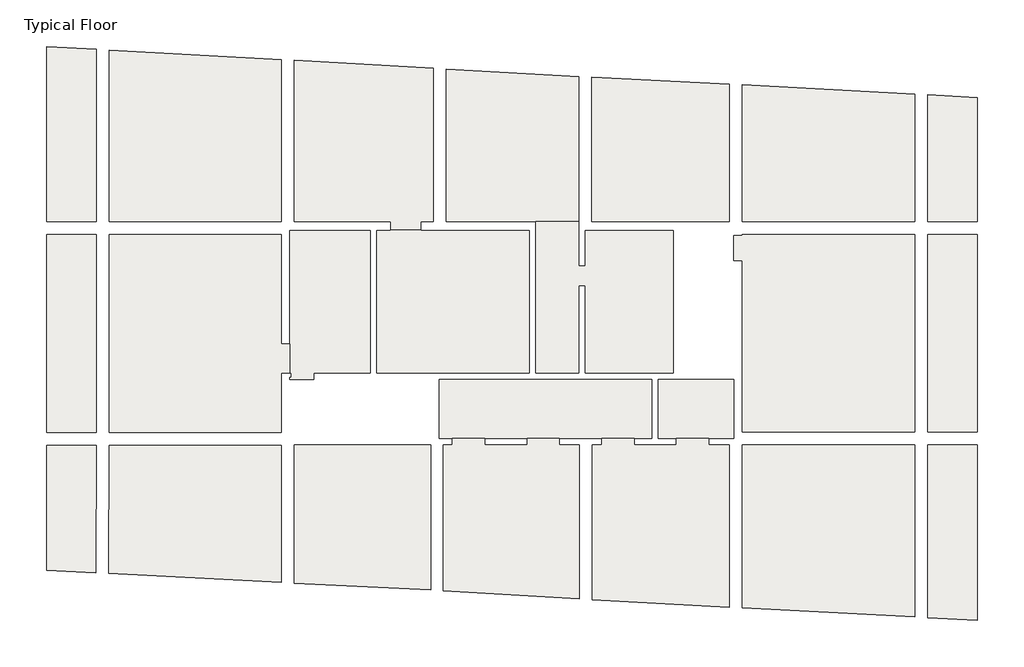
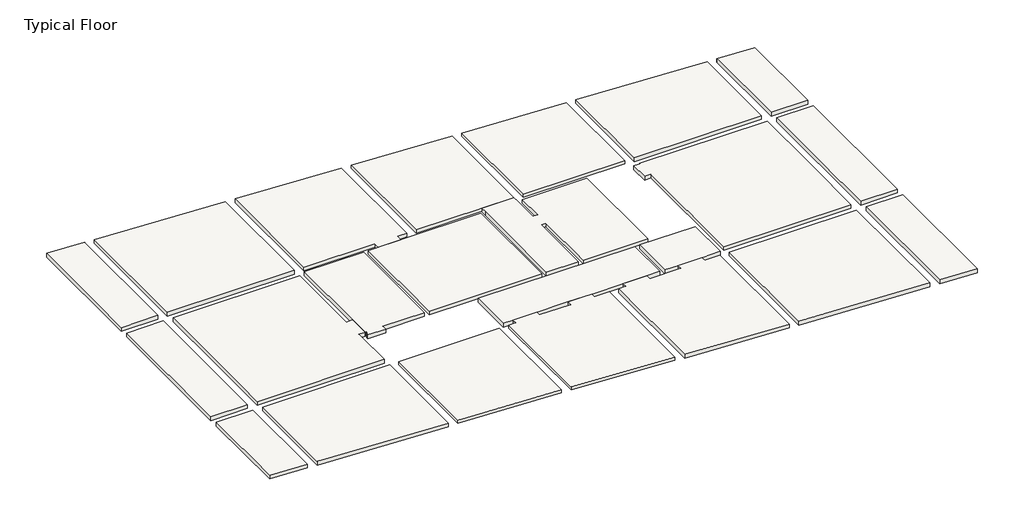
# One storey: 23 slabs.
"""IFC4 building model written with IfcOpenShell, lengths in millimetres."""

from ifc_helpers import new_model, si_unit, frame, origin, place, context, project, spatial, polyline, outline, extrude, faceted_brep, element, save

model = new_model("IFC4")

# Units and contexts
model_context = context("Model", 3, world=origin())
ifc_project = project(units=[si_unit("LENGTHUNIT", "METRE", prefix="MILLI")], contexts=[model_context])

# Site, building, storey
site = spatial("IfcSite", under=ifc_project)
building = spatial("IfcBuilding", under=site)
storey = spatial("IfcBuildingStorey", under=building, Name="Typical Floor", Elevation=3500.0)

# Slabs
placement = place(None, origin())
element("IfcSlab", 1, ObjectType="20", at=placement, inside=storey, context=model_context, shape_type="Brep", body=[
    faceted_brep([(-702.7226745, -8172.2965545, 3300.0), (-702.7226745, -14884.028101, 3300.0), (-6997.0277588, -14575.1203917, 3300.0), (-6997.0277588, -8172.2965545, 3300.0), (-702.7226745, -8172.2965545, 3500.0), (-6997.0277588, -8172.2965545, 3500.0), (-6997.0277588, -14560.7582621, 3500.0), (-6997.0277588, -14575.1203917, 3500.0), (-702.7226745, -14884.028101, 3500.0)], [[[0, 1, 2, 3]], [[4, 5, 6, 7, 8]], [[1, 0, 4, 8]], [[2, 1, 8, 7]], [[3, 2, 7, 6, 5]], [[0, 3, 5, 4]]]),
])
element("IfcSlab", 2, ObjectType="20", at=placement, inside=storey, context=model_context, shape_type="Brep", body=[
    faceted_brep([(-102.7226745, -8172.2965545, 3300.0), (309.3899821, -8172.2965545, 3300.0), (309.3899821, -7872.2965545, 3300.0), (1808.0058991, -7872.2965545, 3300.0), (1808.0058991, -8172.2965545, 3300.0), (3757.0255069, -8172.2965545, 3300.0), (3757.0255069, -7872.2965545, 3300.0), (5255.6414239, -7872.2965545, 3300.0), (5255.6414239, -8172.2965545, 3300.0), (6172.0250706, -8172.2965545, 3300.0), (6172.0250706, -15300.3845543, 3300.0), (-102.7226745, -14916.8878336, 3300.0), (309.3899821, -8172.2965545, 3500.0), (-102.7226745, -8172.2965545, 3500.0), (-102.7226745, -14899.1123715, 3500.0), (-102.7226745, -14916.8878336, 3500.0), (6172.0250706, -15300.3845543, 3500.0), (6172.0250706, -8172.2965545, 3500.0), (5255.6414239, -8172.2965545, 3500.0), (5255.6414239, -7872.2965545, 3500.0), (3757.0255069, -7872.2965545, 3500.0), (3757.0255069, -8172.2965545, 3500.0), (1808.0058991, -8172.2965545, 3500.0), (1808.0058991, -7872.2965545, 3500.0), (309.3899821, -7872.2965545, 3500.0)], [[[0, 1, 2, 3, 4, 5, 6, 7, 8, 9, 10, 11]], [[12, 13, 14, 15, 16, 17, 18, 19, 20, 21, 22, 23, 24]], [[1, 0, 13, 12]], [[2, 1, 12, 24]], [[3, 2, 24, 23]], [[4, 3, 23, 22]], [[5, 4, 22, 21]], [[6, 5, 21, 20]], [[7, 6, 20, 19]], [[8, 7, 19, 18]], [[9, 8, 18, 17]], [[10, 9, 17, 16]], [[11, 10, 16, 15]], [[0, 11, 15, 14, 13]]]),
])
element("IfcSlab", 3, ObjectType="20", at=placement, inside=storey, context=model_context, shape_type="Brep", body=[
    faceted_brep([(6756.4488056, 8818.2924867, 3300.0), (13105.5837537, 8500.9277886, 3300.0), (13105.5837537, 2137.8533878, 3300.0), (6756.4488056, 2137.8533878, 3300.0), (6756.4488056, 8818.2924867, 3500.0), (6756.4488056, 2137.8533878, 3500.0), (13105.5837537, 2137.8533878, 3500.0), (13105.5837537, 8486.6836559, 3500.0), (13105.5837537, 8500.9277886, 3500.0)], [[[0, 1, 2, 3]], [[4, 5, 6, 7, 8]], [[1, 0, 4, 8]], [[2, 1, 8, 7, 6]], [[3, 2, 6, 5]], [[0, 3, 5, 4]]]),
])
element("IfcSlab", 4, ObjectType="20", at=placement, inside=storey, context=model_context, shape_type="Brep", body=[
    faceted_brep([(33.1500744, 9202.9682104, 3300.0), (6156.4488056, 8850.5502029, 3300.0), (6156.4488056, 2137.8533878, 3300.0), (4155.2954031, 2137.8533878, 3300.0), (33.1500744, 2137.8533878, 3300.0), (33.1500744, 9202.9682104, 3500.0), (33.1500744, 2137.8533878, 3500.0), (4155.2954031, 2137.8533878, 3500.0), (4158.2942497, 2137.8533878, 3500.0), (6156.4488056, 2137.8533878, 3500.0), (6156.4488056, 8832.8840986, 3500.0), (6156.4488056, 8850.5502029, 3500.0)], [[[0, 1, 2, 3, 4]], [[5, 6, 7, 8, 9, 10, 11]], [[1, 0, 5, 11]], [[2, 1, 11, 10, 9]], [[4, 3, 7, 6]], [[0, 4, 6, 5]], [[3, 2, 9, 8, 7]]]),
])
element("IfcSlab", 5, ObjectType="25", at=placement, inside=storey, context=model_context, shape_type="Brep", body=[
    faceted_brep([(-7599.5626242, 9632.0768029, 3250.0), (-7599.5626242, 2137.8533878, 3250.0), (-15545.0048536, 2137.8533878, 3250.0), (-15536.4663265, 10078.6836364, 3250.0), (-7599.5626242, 9632.0768029, 3500.0), (-15536.4663265, 10078.6836364, 3500.0), (-15545.0048536, 2137.8533878, 3500.0), (-7599.5626242, 2137.8533878, 3500.0), (-7599.5626242, 9596.3425232, 3500.0)], [[[0, 1, 2, 3]], [[4, 5, 6, 7, 8]], [[1, 0, 4, 8, 7]], [[2, 1, 7, 6]], [[3, 2, 6, 5]], [[0, 3, 5, 4]]]),
])
element("IfcSlab", 6, ObjectType="25", at=placement, inside=storey, context=model_context, shape_type="Brep", body=[
    faceted_brep([(-16136.4303725, 10112.4434063, 3250.0), (-16145.0052005, 2137.8533878, 3250.0), (-18443.7818749, 2137.8533878, 3250.0), (-18443.7818749, 10242.2772794, 3250.0), (-16136.4303725, 10112.4434063, 3500.0), (-18443.7818749, 10242.2772794, 3500.0), (-18443.7818749, 2137.8533878, 3500.0), (-16145.0052005, 2137.8533878, 3500.0), (-16136.4525662, 10091.8032303, 3500.0)], [[[0, 1, 2, 3]], [[4, 5, 6, 7, 8]], [[1, 0, 4, 8, 7]], [[2, 1, 7, 6]], [[3, 2, 6, 5]], [[0, 3, 5, 4]]]),
])
element("IfcSlab", 7, ObjectType="25", at=placement, inside=storey, context=model_context, shape_type="Brep", body=[
    faceted_brep([(-16155.474628, -7598.714204, 3250.0), (-18443.7818749, -7598.714204, 3250.0), (-18443.7818749, 1537.8533878, 3250.0), (-16145.6503618, 1537.8533878, 3250.0), (-16150.3278096, -2812.1730545, 3250.0), (-16150.9729705, -3412.1727076, 3250.0), (-16155.4742813, -7598.391797, 3250.0), (-18443.7818749, -7598.714204, 3500.0), (-16155.474628, -7598.714204, 3500.0), (-16155.4742813, -7598.391797, 3500.0), (-16150.9729705, -3412.1727076, 3500.0), (-16150.3278096, -2812.1730545, 3500.0), (-16145.6503618, 1537.8533878, 3500.0), (-18443.7818749, 1537.8533878, 3500.0)], [[[0, 1, 2, 3, 4, 5, 6]], [[7, 8, 9, 10, 11, 12, 13]], [[8, 0, 6, 5, 4, 3, 12, 11, 10, 9]], [[1, 0, 8, 7]], [[2, 1, 7, 13]], [[3, 2, 13, 12]]]),
])
element("IfcSlab", 8, ObjectType="25", at=placement, inside=storey, context=model_context, shape_type="SweptSolid", body=[
    extrude(outline(polyline([(-18443.7818749, -8198.714204), (-16156.1197893, -8198.714204), (-16162.4537125, -14089.2628163), (-18443.7818749, -13968.0424313), (-18443.7818749, -8198.714204)])), frame((0.0, 0.0, 3250.0), z_axis=(0.0, 0.0, 1.0), x_axis=(1.0, 0.0, 0.0)), (0.0, 0.0, 1.0), 250.0),
])
element("IfcSlab", 9, ObjectType="25", at=placement, inside=storey, context=model_context, shape_type="Brep", body=[
    faceted_brep([(-7597.0277588, -14544.3942826, 3250.0), (-15562.4876449, -14121.1425427, 3250.0), (-15556.1197891, -8199.036611, 3250.0), (-15556.1194424, -8198.714204, 3250.0), (-7597.0277588, -8198.714204, 3250.0), (-15562.4876449, -14121.1425427, 3500.0), (-7597.0277588, -14544.3942826, 3500.0), (-7597.0277588, -8198.714204, 3500.0), (-15556.1194424, -8198.714204, 3500.0), (-15556.1197891, -8199.036611, 3500.0), (-15562.471289, -14105.9314844, 3500.0)], [[[0, 1, 2, 3, 4]], [[5, 6, 7, 8, 9, 10]], [[1, 0, 6, 5]], [[1, 5, 10, 9, 8, 3, 2]], [[4, 3, 8, 7]], [[0, 4, 7, 6]]]),
])
element("IfcSlab", 10, ObjectType="25", at=placement, inside=storey, context=model_context, shape_type="Brep", body=[
    faceted_brep([(-7599.5626242, 1537.8533878, 3250.0), (-7599.5626242, -3512.6656433, 3250.0), (-7199.5626242, -3512.6656433, 3250.0), (-7199.5626242, -4855.687558, 3250.0), (-7599.5626242, -4855.687558, 3250.0), (-7599.5626242, -5055.687558, 3250.0), (-7599.5626242, -7598.714204, 3250.0), (-15555.4742811, -7598.714204, 3250.0), (-15550.9733173, -3412.8178686, 3250.0), (-15550.3281564, -2812.8182154, 3250.0), (-15545.6500149, 1537.8533878, 3250.0), (-7599.5626242, -3512.6656433, 3500.0), (-7599.5626242, 1537.8533878, 3500.0), (-15545.0119134, 1537.8533878, 3500.0), (-15545.6500149, 1537.8533878, 3500.0), (-15550.3281564, -2812.8182154, 3500.0), (-15550.9733173, -3412.8178686, 3500.0), (-15555.4742811, -7598.714204, 3500.0), (-7599.5626242, -7598.714204, 3500.0), (-7599.5626242, -5055.687558, 3500.0), (-7599.5626242, -4855.687558, 3500.0), (-7199.5626242, -4855.687558, 3500.0), (-7199.5626242, -3512.6656433, 3500.0)], [[[0, 1, 2, 3, 4, 5, 6, 7, 8, 9, 10]], [[11, 12, 13, 14, 15, 16, 17, 18, 19, 20, 21, 22]], [[1, 0, 12, 11]], [[2, 1, 11, 22]], [[3, 2, 22, 21]], [[4, 3, 21, 20]], [[4, 20, 19, 18, 6, 5]], [[7, 6, 18, 17]], [[7, 17, 16, 15, 14, 10, 9, 8]], [[0, 10, 14, 13, 12]]]),
])
element("IfcSlab", 11, ObjectType="25", at=placement, inside=storey, context=model_context, shape_type="Brep", body=[
    faceted_brep([(-3490.3793374, 1737.8533878, 3250.0), (-3490.3793374, -4855.687558, 3250.0), (-6094.5315865, -4855.687558, 3250.0), (-6094.5315865, -5155.687558, 3250.0), (-7199.5626242, -5155.687558, 3250.0), (-7199.5626242, -5055.687558, 3250.0), (-7139.5626242, -5055.687558, 3250.0), (-7139.5626242, -4855.687558, 3250.0), (-7199.5626242, -4855.687558, 3250.0), (-7199.5626242, -3512.6656433, 3250.0), (-7199.5626242, 1737.8533878, 3250.0), (-3490.3793374, -4855.687558, 3500.0), (-3490.3793374, 1737.8533878, 3500.0), (-7199.5626242, 1737.8533878, 3500.0), (-7199.5626242, -3512.6656433, 3500.0), (-7199.5626242, -4855.687558, 3500.0), (-7139.5626242, -4855.687558, 3500.0), (-7139.5626242, -5055.687558, 3500.0), (-7199.5626242, -5055.687558, 3500.0), (-7199.5626242, -5155.687558, 3500.0), (-6094.5315865, -5155.687558, 3500.0), (-6094.5315865, -4855.687558, 3500.0)], [[[0, 1, 2, 3, 4, 5, 6, 7, 8, 9, 10]], [[11, 12, 13, 14, 15, 16, 17, 18, 19, 20, 21]], [[1, 0, 12, 11]], [[2, 1, 11, 21]], [[3, 2, 21, 20]], [[4, 3, 20, 19]], [[5, 4, 19, 18]], [[6, 5, 18, 17]], [[7, 6, 17, 16]], [[8, 7, 16, 15]], [[10, 9, 8, 15, 14, 13]], [[0, 10, 13, 12]]]),
])
element("IfcSlab", 12, ObjectType="25", at=placement, inside=storey, context=model_context, shape_type="Brep", body=[
    faceted_brep([(6772.0250706, -8172.2965545, 3250.0), (7204.6610317, -8172.2965545, 3250.0), (7204.6610317, -7872.2965545, 3250.0), (8703.2769487, -7872.2965545, 3250.0), (8703.2769487, -8172.2965545, 3250.0), (10652.2965565, -8172.2965545, 3250.0), (10652.2965565, -7872.2965545, 3250.0), (12150.9124735, -7872.2965545, 3250.0), (12150.9124735, -8172.2965545, 3250.0), (13105.5837537, -8172.2965545, 3250.0), (13105.5837537, -15690.2789818, 3250.0), (6772.0250706, -15335.6091222, 3250.0), (7204.6610317, -8172.2965545, 3500.0), (6772.0250706, -8172.2965545, 3500.0), (6772.0250706, -15319.2795755, 3500.0), (6772.0250706, -15335.6091222, 3500.0), (13105.5837537, -15690.2789818, 3500.0), (13105.5837537, -8172.2965545, 3500.0), (12150.9124735, -8172.2965545, 3500.0), (12150.9124735, -7872.2965545, 3500.0), (10652.2965565, -7872.2965545, 3500.0), (10652.2965565, -8172.2965545, 3500.0), (8703.2769487, -8172.2965545, 3500.0), (8703.2769487, -7872.2965545, 3500.0), (7204.6610317, -7872.2965545, 3500.0)], [[[0, 1, 2, 3, 4, 5, 6, 7, 8, 9, 10, 11]], [[12, 13, 14, 15, 16, 17, 18, 19, 20, 21, 22, 23, 24]], [[1, 0, 13, 12]], [[2, 1, 12, 24]], [[3, 2, 24, 23]], [[4, 3, 23, 22]], [[5, 4, 22, 21]], [[6, 5, 21, 20]], [[7, 6, 20, 19]], [[8, 7, 19, 18]], [[9, 8, 18, 17]], [[10, 9, 17, 16]], [[11, 10, 16, 15]], [[0, 11, 15, 14, 13]]]),
])
element("IfcSlab", 13, ObjectType="25", at=placement, inside=storey, context=model_context, shape_type="Brep", body=[
    faceted_brep([(9530.3819083, -5155.687558, 3250.0), (9530.3819083, -7872.2965545, 3250.0), (8703.2769487, -7872.2965545, 3250.0), (7204.6610317, -7872.2965545, 3250.0), (-291.6077111, -7872.2965545, 3250.0), (-291.6077111, -5155.687558, 3250.0), (9530.3819083, -5155.687558, 3500.0), (-291.6077111, -5155.687558, 3500.0), (-291.6077111, -7872.2965545, 3500.0), (309.3899821, -7872.2965545, 3500.0), (1808.0058991, -7872.2965545, 3500.0), (3757.0255069, -7872.2965545, 3500.0), (5255.6414239, -7872.2965545, 3500.0), (7204.6610317, -7872.2965545, 3500.0), (8703.2769487, -7872.2965545, 3500.0), (9530.3819083, -7872.2965545, 3500.0)], [[[0, 1, 2, 3, 4, 5]], [[6, 7, 8, 9, 10, 11, 12, 13, 14, 15]], [[1, 0, 6, 15]], [[4, 3, 2, 1, 15, 14, 13, 12, 11, 10, 9, 8]], [[5, 4, 8, 7]], [[0, 5, 7, 6]]]),
])
element("IfcSlab", 14, ObjectType="25", at=placement, inside=storey, context=model_context, shape_type="Brep", body=[
    faceted_brep([(13305.5837537, -5155.687558, 3250.0), (13305.5837537, -7872.2965545, 3250.0), (12150.9124735, -7872.2965545, 3250.0), (10652.2965565, -7872.2965545, 3250.0), (9830.3819083, -7872.2965545, 3250.0), (9830.3819083, -5155.687558, 3250.0), (13305.5837537, -5155.687558, 3500.0), (9830.3819083, -5155.687558, 3500.0), (9830.3819083, -7872.2965545, 3500.0), (10652.2965565, -7872.2965545, 3500.0), (12150.9124735, -7872.2965545, 3500.0), (13305.5837537, -7872.2965545, 3500.0)], [[[0, 1, 2, 3, 4, 5]], [[6, 7, 8, 9, 10, 11]], [[1, 0, 6, 11]], [[4, 3, 2, 1, 11, 10, 9, 8]], [[5, 4, 8, 7]], [[0, 5, 7, 6]]]),
])
element("IfcSlab", 15, ObjectType="25", at=placement, inside=storey, context=model_context, shape_type="Brep", body=[
    faceted_brep([(13305.5837537, 1490.9099045, 3250.0), (13705.5837537, 1490.9099045, 3250.0), (13705.5837537, 1537.8533878, 3250.0), (21672.320563, 1537.8533878, 3250.0), (21672.320563, -7572.2965545, 3250.0), (13705.5837537, -7572.2965545, 3250.0), (13705.5837537, 336.2386242, 3250.0), (13305.5837537, 336.2386242, 3250.0), (13705.5837537, 1490.9099045, 3500.0), (13305.5837537, 1490.9099045, 3500.0), (13305.5837537, 336.2386242, 3500.0), (13705.5837537, 336.2386242, 3500.0), (13705.5837537, -7572.2965545, 3500.0), (21672.320563, -7572.2965545, 3500.0), (21672.320563, -3412.4954615, 3500.0), (21672.320563, -2812.4954615, 3500.0), (21672.320563, 1537.8533878, 3500.0), (13705.5837537, 1537.8533878, 3500.0)], [[[0, 1, 2, 3, 4, 5, 6, 7]], [[8, 9, 10, 11, 12, 13, 14, 15, 16, 17]], [[1, 0, 9, 8]], [[2, 1, 8, 17]], [[3, 2, 17, 16]], [[4, 3, 16, 15, 14, 13]], [[5, 4, 13, 12]], [[6, 5, 12, 11]], [[7, 6, 11, 10]], [[0, 7, 10, 9]]]),
])
element("IfcSlab", 16, ObjectType="25", at=placement, inside=storey, context=model_context, shape_type="SweptSolid", body=[
    extrude(outline(polyline([(13705.5837537, -8172.2965545), (21672.320563, -8172.2965545), (21672.320563, -16132.9877815), (13705.5837537, -15722.5717744), (13705.5837537, -8172.2965545)])), frame((0.0, 0.0, 3250.0), z_axis=(0.0, 0.0, 1.0), x_axis=(1.0, 0.0, 0.0)), (0.0, 0.0, 1.0), 250.0),
])
element("IfcSlab", 17, ObjectType="25", at=placement, inside=storey, context=model_context, shape_type="Brep", body=[
    faceted_brep([(24568.7448881, -16282.2005564, 3250.0), (22272.320563, -16163.8975015, 3250.0), (22272.320563, -8172.2965545, 3250.0), (24568.7448881, -8172.2965545, 3250.0), (24568.7448881, -16282.2005564, 3500.0), (24568.7448881, -8172.2965545, 3500.0), (22272.320563, -8172.2965545, 3500.0), (22272.320563, -16148.8404655, 3500.0), (22272.320563, -16163.8975015, 3500.0)], [[[0, 1, 2, 3]], [[4, 5, 6, 7, 8]], [[1, 0, 4, 8]], [[2, 1, 8, 7, 6]], [[3, 2, 6, 5]], [[0, 3, 5, 4]]]),
])
element("IfcSlab", 18, ObjectType="25", at=placement, inside=storey, context=model_context, shape_type="Brep", body=[
    faceted_brep([(24568.7448881, 1537.8533878, 3250.0), (24568.7448881, -7572.2965545, 3250.0), (22272.320563, -7572.2965545, 3250.0), (22272.320563, 1537.8533878, 3250.0), (24568.7448881, 1537.8533878, 3500.0), (22272.320563, 1537.8533878, 3500.0), (22272.320563, -2812.4954615, 3500.0), (22272.320563, -3412.4954615, 3500.0), (22272.320563, -7572.2965545, 3500.0), (24568.7448881, -7572.2965545, 3500.0)], [[[0, 1, 2, 3]], [[4, 5, 6, 7, 8, 9]], [[1, 0, 4, 9]], [[2, 1, 9, 8]], [[3, 2, 8, 7, 6, 5]], [[0, 3, 5, 4]]]),
])
element("IfcSlab", 19, ObjectType="25", at=placement, inside=storey, context=model_context, shape_type="SweptSolid", body=[
    extrude(outline(polyline([(24568.7448881, 2137.8533878), (22272.320563, 2137.8533878), (22272.320563, 7998.3813629), (22272.7386809, 7998.381946), (22272.7208607, 8011.159025), (24568.7448881, 7885.5038131), (24568.7448881, 2137.8533878)])), frame((0.0, 0.0, 3250.0), z_axis=(0.0, 0.0, 1.0), x_axis=(1.0, 0.0, 0.0)), (0.0, 0.0, 1.0), 250.0),
])
element("IfcSlab", 20, ObjectType="25", at=placement, inside=storey, context=model_context, shape_type="Brep", body=[
    faceted_brep([(10507.8905588, 1737.8533878, 3250.0), (10507.8905588, -4855.687558, 3250.0), (6456.4488056, -4855.687558, 3250.0), (6456.4488056, -810.243498, 3250.0), (6156.4488056, -810.243498, 3250.0), (6156.4488056, -4855.687558, 3250.0), (4155.2954031, -4855.687558, 3250.0), (4155.2954031, 1737.8533878, 3250.0), (4158.2942497, 1737.8533878, 3250.0), (4158.2942497, 2137.8533878, 3250.0), (6156.4488056, 2137.8533878, 3250.0), (6156.4488056, 1737.8533878, 3250.0), (6156.4488056, 90.5638838, 3250.0), (6456.4488056, 90.5638838, 3250.0), (6456.4488056, 1737.8533878, 3250.0), (10507.8905588, -4855.687558, 3500.0), (10507.8905588, 1737.8533878, 3500.0), (6456.4488056, 1737.8533878, 3500.0), (6456.4488056, 90.5638838, 3500.0), (6156.4488056, 90.5638838, 3500.0), (6156.4488056, 1737.8533878, 3500.0), (6156.4488056, 2137.8533878, 3500.0), (4158.2942497, 2137.8533878, 3500.0), (4158.2942497, 1737.8533878, 3500.0), (4155.2954031, 1737.8533878, 3500.0), (4155.2954031, -4855.687558, 3500.0), (6156.4488056, -4855.687558, 3500.0), (6156.4488056, -810.243498, 3500.0), (6456.4488056, -810.243498, 3500.0), (6456.4488056, -4855.687558, 3500.0), (6156.4488056, 2137.8533878, 3300.0)], [[[0, 1, 2, 3, 4, 5, 6, 7, 8, 9, 10, 11, 12, 13, 14]], [[15, 16, 17, 18, 19, 20, 21, 22, 23, 24, 25, 26, 27, 28, 29]], [[1, 0, 16, 15]], [[2, 1, 15, 29]], [[3, 2, 29, 28]], [[0, 14, 17, 16]], [[4, 3, 28, 27]], [[5, 4, 27, 26]], [[6, 5, 26, 25]], [[6, 25, 24, 7]], [[21, 30, 10, 9, 22]], [[10, 30, 21, 20, 19, 12, 11]], [[13, 12, 19, 18]], [[14, 13, 18, 17]], [[23, 8, 7, 24]], [[8, 23, 22, 9]]]),
])
element("IfcSlab", 21, ObjectType="25", at=placement, inside=storey, context=model_context, shape_type="SweptSolid", body=[
    extrude(outline(polyline([(3855.2954031, -4855.687558), (-3190.3793374, -4855.687558), (-3190.3793374, 1737.8533878), (-2548.6261655, 1737.8533878), (-2548.6261655, 1752.8533878), (-1148.2801448, 1752.8533878), (-1148.2801448, 1737.8533878), (3855.2954031, 1737.8533878), (3855.2954031, -4855.687558)])), frame((0.0, 0.0, 3250.0), z_axis=(0.0, 0.0, 1.0), x_axis=(1.0, 0.0, 0.0)), (0.0, 0.0, 1.0), 250.0),
])
element("IfcSlab", 22, ObjectType="25", at=placement, inside=storey, context=model_context, shape_type="SweptSolid", body=[
    extrude(outline(polyline([(13705.5837537, 8480.0153679), (21672.320563, 8044.0173164), (21672.320563, 2137.8533878), (13705.5837537, 2137.8533878), (13705.5837537, 8480.0153679)])), frame((0.0, 0.0, 3250.0), z_axis=(0.0, 0.0, 1.0), x_axis=(1.0, 0.0, 0.0)), (0.0, 0.0, 1.0), 250.0),
])
element("IfcSlab", 23, ObjectType="25", at=placement, inside=storey, context=model_context, shape_type="Brep", body=[
    faceted_brep([(-566.8499256, 9237.1370793, 3250.0), (-566.8499256, 2137.8533878, 3250.0), (-1148.2801448, 2137.8533878, 3250.0), (-1148.2801448, 1752.8533878, 3250.0), (-2548.6261655, 1752.8533878, 3250.0), (-2548.6261655, 2137.8533878, 3250.0), (-6999.5626242, 2137.8533878, 3250.0), (-6999.5626242, 9599.1036038, 3250.0), (-566.8499256, 2137.8533878, 3500.0), (-566.8499256, 9220.7307485, 3500.0), (-566.8499256, 9237.1370793, 3500.0), (-6999.5626242, 9599.1036038, 3500.0), (-6999.5626242, 9596.3425232, 3500.0), (-6999.5626242, 2137.8533878, 3500.0), (-2548.6261655, 2137.8533878, 3500.0), (-2548.6261655, 1752.8533878, 3500.0), (-1148.2801448, 1752.8533878, 3500.0), (-1148.2801448, 2137.8533878, 3500.0)], [[[0, 1, 2, 3, 4, 5, 6, 7]], [[8, 9, 10, 11, 12, 13, 14, 15, 16, 17]], [[1, 0, 10, 9, 8]], [[2, 1, 8, 17]], [[2, 17, 16, 3]], [[14, 5, 4, 15]], [[6, 5, 14, 13]], [[7, 6, 13, 12, 11]], [[0, 7, 11, 10]], [[4, 3, 16, 15]]]),
])

save(model, "model.ifc")

# Revit data of these elements
# Type "20"
#   Function = 0
#   Layers, outside or top first: 20 cm "Concrete" (function 1)
# Type "25"
#   Function = 0
#   Layers, outside or top first: 25 cm "Concrete" (function 1)
# Element 1 (IfcSlab, "20")
#   Mark = "S20"
#   SOFiSTiK_AMG_Comments = ""
#   Height Offset From Level = 0 cm
#   built-in parameter 1001954 = 1
#   SOFiSTiK_AMG_Scheduled = yes
#   SOFiSTiK_AMG_Adjusted = yes
#   Phase Created = New Construction
#   Materials on its faces: "Concrete"
# Element 2 (IfcSlab, "20")
#   Mark = "S21"
#   SOFiSTiK_AMG_Comments = ""
#   built-in parameter 1001955 = 1.5708 (stored number, unit not read)
#   Height Offset From Level = 0 cm
#   built-in parameter 1001954 = 1
#   SOFiSTiK_AMG_Scheduled = yes
#   SOFiSTiK_AMG_Adjusted = yes
#   Phase Created = New Construction
#   Materials on its faces: "Concrete"
# Element 3 (IfcSlab, "20")
#   Mark = "S22"
#   SOFiSTiK_AMG_Comments = ""
#   built-in parameter 1001955 = 1.5708 (stored number, unit not read)
#   Height Offset From Level = 0 cm
#   built-in parameter 1001954 = 1
#   SOFiSTiK_AMG_Scheduled = yes
#   SOFiSTiK_AMG_Adjusted = yes
#   Phase Created = New Construction
#   Materials on its faces: "Concrete"
# Element 4 (IfcSlab, "20")
#   Mark = "S23"
#   SOFiSTiK_AMG_Comments = ""
#   built-in parameter 1001955 = 1.5708 (stored number, unit not read)
#   Height Offset From Level = 0 cm
#   built-in parameter 1001954 = 1
#   SOFiSTiK_AMG_Scheduled = yes
#   SOFiSTiK_AMG_Adjusted = yes
#   Phase Created = New Construction
#   Materials on its faces: "Concrete"
# Element 5 (IfcSlab, "25")
#   Mark = "S1"
#   SOFiSTiK_AMG_Comments = ""
#   built-in parameter 1001955 = -0.0562104 (stored number, unit not read)
#   Height Offset From Level = 0 cm
#   built-in parameter 1001954 = 1
#   SOFiSTiK_AMG_Scheduled = yes
#   SOFiSTiK_AMG_Adjusted = yes
#   Phase Created = New Construction
#   Materials on its faces: "Concrete"
# Element 6 (IfcSlab, "25")
#   Mark = "S2"
#   SOFiSTiK_AMG_Comments = ""
#   built-in parameter 1001955 = -0.0562104 (stored number, unit not read)
#   Height Offset From Level = 0 cm
#   built-in parameter 1001954 = 1
#   SOFiSTiK_AMG_Scheduled = yes
#   SOFiSTiK_AMG_Adjusted = yes
#   Phase Created = New Construction
#   Materials on its faces: "Concrete"
# Element 7 (IfcSlab, "25")
#   Mark = "S3"
#   SOFiSTiK_AMG_Comments = ""
#   Height Offset From Level = 0 cm
#   built-in parameter 1001954 = 1
#   SOFiSTiK_AMG_Scheduled = yes
#   SOFiSTiK_AMG_Adjusted = yes
#   Phase Created = New Construction
#   Materials on its faces: "Concrete"
# Element 8 (IfcSlab, "25")
#   Mark = "S4"
#   SOFiSTiK_AMG_Comments = ""
#   built-in parameter 1001955 = 1.5708 (stored number, unit not read)
#   Height Offset From Level = 0 cm
#   built-in parameter 1001954 = 1
#   SOFiSTiK_AMG_Scheduled = yes
#   SOFiSTiK_AMG_Adjusted = yes
#   Phase Created = New Construction
#   Materials on its faces: "Concrete"
# Element 9 (IfcSlab, "25")
#   Mark = "S5"
#   SOFiSTiK_AMG_Comments = ""
#   built-in parameter 1001955 = -0.053086 (stored number, unit not read)
#   Height Offset From Level = 0 cm
#   built-in parameter 1001954 = 1
#   SOFiSTiK_AMG_Scheduled = yes
#   SOFiSTiK_AMG_Adjusted = yes
#   Phase Created = New Construction
#   Materials on its faces: "Concrete"
# Element 10 (IfcSlab, "25")
#   Mark = "S6"
#   SOFiSTiK_AMG_Comments = ""
#   Height Offset From Level = 0 cm
#   built-in parameter 1001954 = 1
#   SOFiSTiK_AMG_Scheduled = yes
#   SOFiSTiK_AMG_Adjusted = yes
#   Phase Created = New Construction
#   Materials on its faces: "Concrete"
# Element 11 (IfcSlab, "25")
#   Mark = "S7"
#   SOFiSTiK_AMG_Comments = ""
#   Height Offset From Level = 0 cm
#   built-in parameter 1001954 = 1
#   SOFiSTiK_AMG_Scheduled = yes
#   SOFiSTiK_AMG_Adjusted = yes
#   Phase Created = New Construction
#   Materials on its faces: "Concrete"
# Element 12 (IfcSlab, "25")
#   Mark = "S8"
#   SOFiSTiK_AMG_Comments = ""
#   built-in parameter 1001955 = 1.5708 (stored number, unit not read)
#   Height Offset From Level = 0 cm
#   built-in parameter 1001954 = 1
#   SOFiSTiK_AMG_Scheduled = yes
#   SOFiSTiK_AMG_Adjusted = yes
#   Phase Created = New Construction
#   Materials on its faces: "Concrete"
# Element 13 (IfcSlab, "25")
#   Mark = "S9"
#   SOFiSTiK_AMG_Comments = ""
#   Height Offset From Level = 0 cm
#   built-in parameter 1001954 = 1
#   SOFiSTiK_AMG_Scheduled = yes
#   SOFiSTiK_AMG_Adjusted = yes
#   Phase Created = New Construction
#   Materials on its faces: "Concrete"
# Element 14 (IfcSlab, "25")
#   Mark = "S10"
#   SOFiSTiK_AMG_Comments = ""
#   Height Offset From Level = 0 cm
#   built-in parameter 1001954 = 1
#   SOFiSTiK_AMG_Scheduled = yes
#   SOFiSTiK_AMG_Adjusted = yes
#   Phase Created = New Construction
#   Materials on its faces: "Concrete"
# Element 15 (IfcSlab, "25")
#   Mark = "S11"
#   SOFiSTiK_AMG_Comments = ""
#   built-in parameter 1001955 = 1.5708 (stored number, unit not read)
#   Height Offset From Level = 0 cm
#   built-in parameter 1001954 = 1
#   SOFiSTiK_AMG_Scheduled = yes
#   SOFiSTiK_AMG_Adjusted = yes
#   Phase Created = New Construction
#   Materials on its faces: "Concrete"
# Element 16 (IfcSlab, "25")
#   Mark = "S12"
#   SOFiSTiK_AMG_Comments = ""
#   built-in parameter 1001955 = 1.5708 (stored number, unit not read)
#   Height Offset From Level = 0 cm
#   built-in parameter 1001954 = 1
#   SOFiSTiK_AMG_Scheduled = yes
#   SOFiSTiK_AMG_Adjusted = yes
#   Phase Created = New Construction
#   Materials on its faces: "Concrete"
# Element 17 (IfcSlab, "25")
#   Mark = "S13"
#   SOFiSTiK_AMG_Comments = ""
#   built-in parameter 1001955 = -0.0514707 (stored number, unit not read)
#   Height Offset From Level = 0 cm
#   built-in parameter 1001954 = 1
#   SOFiSTiK_AMG_Scheduled = yes
#   SOFiSTiK_AMG_Adjusted = yes
#   Phase Created = New Construction
#   Materials on its faces: "Concrete"
# Element 18 (IfcSlab, "25")
#   Mark = "S14"
#   SOFiSTiK_AMG_Comments = ""
#   Height Offset From Level = 0 cm
#   built-in parameter 1001954 = 1
#   SOFiSTiK_AMG_Scheduled = yes
#   SOFiSTiK_AMG_Adjusted = yes
#   Phase Created = New Construction
#   Materials on its faces: "Concrete"
# Element 19 (IfcSlab, "25")
#   Mark = "S15"
#   SOFiSTiK_AMG_Comments = ""
#   built-in parameter 1001955 = -1.5708 (stored number, unit not read)
#   Height Offset From Level = 0 cm
#   built-in parameter 1001954 = 1
#   SOFiSTiK_AMG_Scheduled = yes
#   SOFiSTiK_AMG_Adjusted = yes
#   Phase Created = New Construction
#   Materials on its faces: "Concrete"
# Element 20 (IfcSlab, "25")
#   Mark = "S16"
#   SOFiSTiK_AMG_Comments = ""
#   Height Offset From Level = 0 cm
#   built-in parameter 1001954 = 1
#   SOFiSTiK_AMG_Scheduled = yes
#   SOFiSTiK_AMG_Adjusted = yes
#   Phase Created = New Construction
#   Materials on its faces: "Concrete"
# Element 21 (IfcSlab, "25")
#   Mark = "S17"
#   SOFiSTiK_AMG_Comments = ""
#   Height Offset From Level = 0 cm
#   built-in parameter 1001954 = 1
#   SOFiSTiK_AMG_Scheduled = yes
#   SOFiSTiK_AMG_Adjusted = yes
#   Phase Created = New Construction
#   Materials on its faces: "Concrete"
# Element 22 (IfcSlab, "25")
#   Mark = "S18"
#   SOFiSTiK_AMG_Comments = ""
#   built-in parameter 1001955 = 1.5708 (stored number, unit not read)
#   Height Offset From Level = 0 cm
#   built-in parameter 1001954 = 1
#   SOFiSTiK_AMG_Scheduled = yes
#   SOFiSTiK_AMG_Adjusted = yes
#   Phase Created = New Construction
#   Materials on its faces: "Concrete"
# Element 23 (IfcSlab, "25")
#   Mark = "S19"
#   SOFiSTiK_AMG_Comments = ""
#   built-in parameter 1001955 = -0.0562104 (stored number, unit not read)
#   Height Offset From Level = 0 cm
#   built-in parameter 1001954 = 1
#   SOFiSTiK_AMG_Scheduled = yes
#   SOFiSTiK_AMG_Adjusted = yes
#   Phase Created = New Construction
#   Materials on its faces: "Concrete"
# Materials
#   "Concrete": class "Concrete", colour RGB 192 192 192, transparency 0, Keynote = "01000", Description = "Cast-in-place concrete", Cost = 0
